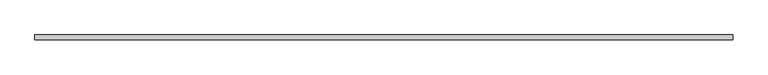
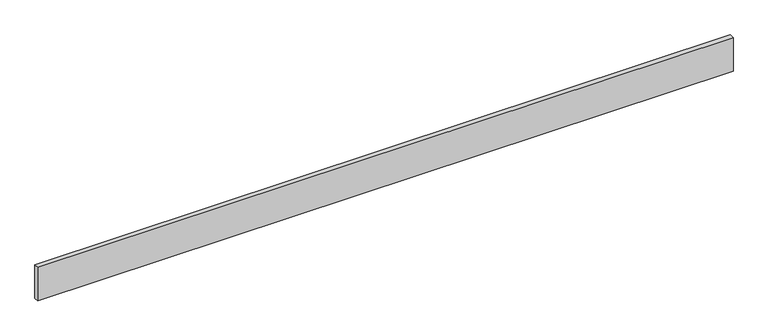
"""IFC4 building model written with IfcOpenShell, lengths in millimetres: proxy geometry, Footer002 : Footer002."""

from ifc_helpers import new_model, si_unit, frame, origin, place, context, project, spatial, polyline, outline, extrude, source, transform, mapped, element, save


def generic_models_6f2e6af7(model_context):
    return source(origin(), model_context, "Body", "SweptSolid", [
        extrude(outline(polyline([(12383.0178845, -4235.9042972), (12383.0178845, -4222.1253493), (14383.0178845, -4222.1253493), (14383.0178845, -4235.9042972), (12383.0178845, -4235.9042972)])), frame((0.0, 0.0, 40150.796), z_axis=(0.0, 0.0, 1.0), x_axis=(1.0, 0.0, 0.0)), (0.0, 0.0, 1.0), 101.6),
    ])


if __name__ == "__main__":
    model = new_model("IFC4")
    model_context = context("Model", 3, world=origin())
    ifc_project = project(units=[si_unit("LENGTHUNIT", "METRE", prefix="MILLI")], contexts=[model_context])
    site = spatial("IfcSite", under=ifc_project)
    building = spatial("IfcBuilding", under=site)
    placement = place(None, origin())
    generic_models_shape = generic_models_6f2e6af7(model_context)
    element("IfcBuildingElementProxy", 1, Name="Footer002 : Footer002", ObjectType="Footer002 : Footer002", at=placement, inside=building, context=model_context, shape_type="MappedRepresentation", body=[
        mapped(generic_models_shape, transform((0.0, 0.0, 0.0), x_axis=(1.0, 0.0, 0.0), y_axis=(0.0, 1.0, 0.0), z_axis=(0.0, 0.0, 1.0))),
    ])
    save(model, "model.ifc")

# Revit data of these elements
# Type "Footer002 : Footer002"
#   NameOverride = "Footer002"
# Element 1 (IfcBuildingElementProxy, "Footer002 : Footer002")
#   Materials on its faces: "FOOTER MATERIAL TBD"
# Materials
#   "FOOTER MATERIAL TBD": class "Unassigned", colour RGB 148 103 60, transparency 0
